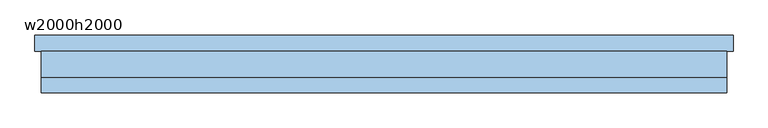
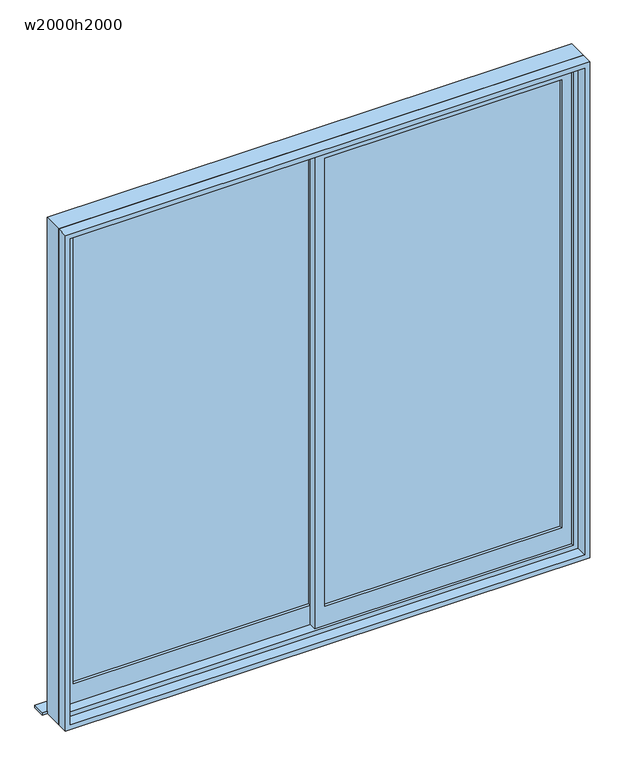
"""IFC4 building model written with IfcOpenShell, lengths in millimetres: window geometry, 引違い掃出窓_2枚 : w2000h2000."""

from ifc_helpers import new_model, si_unit, frame, origin, place, context, project, spatial, polyline, outline, extrude, source, transform, mapped, element, save


def w2000h2000_8e7da428(model_context):
    return source(origin(), model_context, "Body", "SweptSolid", [
        extrude(outline(polyline([(-20.0, 12.5), (-960.0, 12.5), (-960.0, 17.5), (-20.0, 17.5), (-20.0, 12.5)])), frame((0.0, 0.0, 80.0), z_axis=(0.0, 0.0, 1.0), x_axis=(1.0, 0.0, 0.0)), (0.0, 0.0, 1.0), 1880.0),
        extrude(outline(polyline([(960.0, -17.5), (20.0, -17.5), (20.0, -12.5), (960.0, -12.5), (960.0, -17.5)])), frame((0.0, 0.0, 80.0), z_axis=(0.0, 0.0, 1.0), x_axis=(1.0, 0.0, 0.0)), (0.0, 0.0, 1.0), 1880.0),
        extrude(outline(polyline([(2000.0, -20.0), (0.0, -20.0), (0.0, 1000.0), (2000.0, 1000.0), (2000.0, -20.0)]), holes=[polyline([(80.0, 960.0), (80.0, 20.0), (1960.0, 20.0), (1960.0, 960.0), (80.0, 960.0)])]), frame((0.0, -30.0, 0.0), z_axis=(0.0, 1.0, 0.0), x_axis=(0.0, 0.0, 1.0)), (0.0, 0.0, 1.0), 30.0),
        extrude(outline(polyline([(2000.0, -1000.0), (0.0, -1000.0), (0.0, 20.0), (2000.0, 20.0), (2000.0, -1000.0)]), holes=[polyline([(80.0, -20.0), (80.0, -960.0), (1960.0, -960.0), (1960.0, -20.0), (80.0, -20.0)])]), frame((0.0, 0.0, 0.0), z_axis=(0.0, 1.0, 0.0), x_axis=(0.0, 0.0, 1.0)), (0.0, 0.0, 1.0), 30.0),
        extrude(outline(polyline([(1060.0, 90.0), (1060.0, 40.0), (-1060.0, 40.0), (-1060.0, 90.0), (1060.0, 90.0)])), frame((0.0, 0.0, -40.0), z_axis=(0.0, 0.0, 1.0), x_axis=(1.0, 0.0, 0.0)), (0.0, 0.0, 1.0), 10.0),
        extrude(outline(polyline([(2040.0, 1040.0), (2040.0, -1040.0), (-40.0, -1040.0), (-40.0, 1040.0), (2040.0, 1040.0)]), holes=[polyline([(-20.0, -1020.0), (2020.0, -1020.0), (2020.0, 1020.0), (-20.0, 1020.0), (-20.0, -1020.0)])]), frame((0.0, -85.0, 0.0), z_axis=(0.0, 1.0, 0.0), x_axis=(0.0, 0.0, 1.0)), (0.0, 0.0, 1.0), 45.0),
        extrude(outline(polyline([(2040.0, -1040.0), (-40.0, -1040.0), (-40.0, 1040.0), (2040.0, 1040.0), (2040.0, -1040.0)]), holes=[polyline([(2000.0, 1000.0), (0.0, 1000.0), (0.0, -1000.0), (2000.0, -1000.0), (2000.0, 1000.0)])]), frame((0.0, -40.0, 0.0), z_axis=(0.0, 1.0, 0.0), x_axis=(0.0, 0.0, 1.0)), (0.0, 0.0, 1.0), 80.0),
    ])


if __name__ == "__main__":
    model = new_model("IFC4")
    model_context = context("Model", 3, world=origin())
    ifc_project = project(units=[si_unit("LENGTHUNIT", "METRE", prefix="MILLI")], contexts=[model_context])
    site = spatial("IfcSite", under=ifc_project)
    building = spatial("IfcBuilding", under=site)
    placement = place(None, origin())
    w2000h2000_shape = w2000h2000_8e7da428(model_context)
    element("IfcWindow", 1, ObjectType="引違い掃出窓_2枚 : w2000h2000", at=placement, inside=building, context=model_context, shape_type="MappedRepresentation", body=[
        mapped(w2000h2000_shape, transform((0.0, 0.0, 0.0), x_axis=(1.0, 0.0, 0.0), y_axis=(0.0, 1.0, 0.0), z_axis=(0.0, 0.0, 1.0))),
    ])
    save(model, "model.ifc")

# Revit data of these elements
# Type "引違い掃出窓_2枚 : w2000h2000"
#   Construction Type Id = "GSP4R"
#   Analytic Construction = "1/8 インチ ピルキントン一重ガラス"
#   Type Mark = "70"
#   Operation = "ダブル パネル縦"
#   Keynote = "08520.R1"
#   Visual Light Transmittance = 0.9
#   Solar Heat Gain Coefficient = 0.86
#   Heat Transfer Coefficient (U) = 6.7069 W/(m²·K)
#   Height = 2000 mm
#   既定の腰高 = 0 mm
#   Width = 2000 mm
#   額縁見附 = 20 mm
#   額縁ちり = 10 mm
#   サッシ見附 = 40 mm
#   サッシの幅 = 80 mm
#   サッシ額縁 [instance default] = none
#   サッシ本体 [instance default] = none
#   サッシガラス [instance default] = ガラス - 透明
#   Manufacturer = ""
#   Wall Closure = (empty or 0)
#   Model = ""
#   Type Comments = ""
#   Assembly Code = ""
# Element 1 (IfcWindow, "引違い掃出窓_2枚 : w2000h2000")
#   Materials on its faces: "ガラス - 透明"
# Materials
#   "ガラス - 透明": class "ガラス", colour RGB 0 128 192, transparency 0.9, Cost = 0
